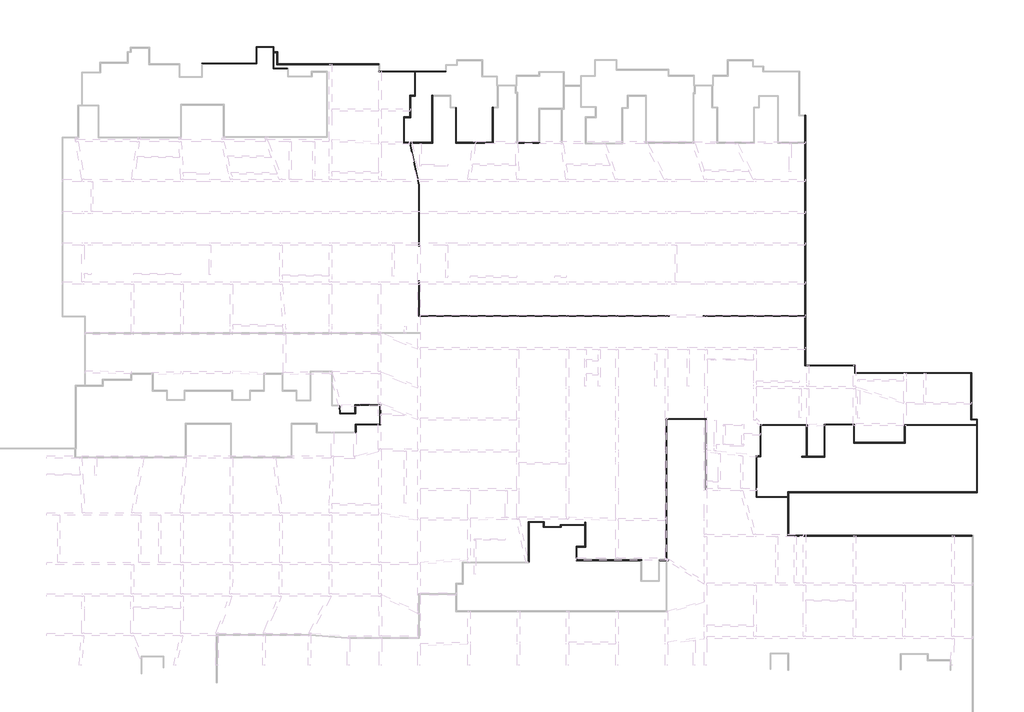
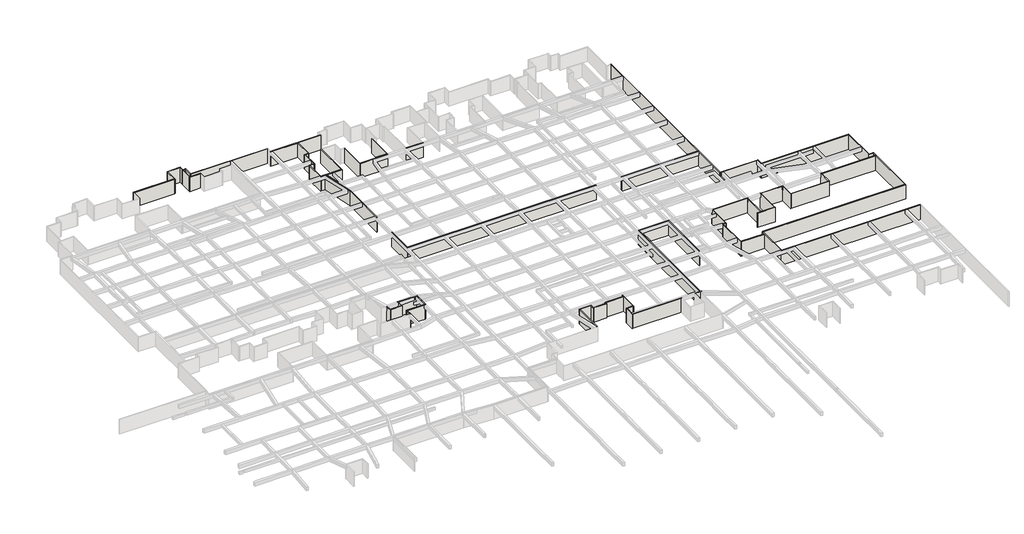
# One storey, part 4 of 16: 70 walls.
"""IFC4 building model written with IfcOpenShell, lengths in millimetres."""

from ifc_helpers import new_model, si_unit, origin, origin_with_axes, place, context, project, spatial, polyline, outline, extrude, faceted_brep, element, save

model = new_model("IFC4")

# Units and contexts
model_context = context("Model", 3, world=origin())
ifc_project = project(units=[si_unit("LENGTHUNIT", "METRE", prefix="MILLI")], contexts=[model_context])

# Site, building, storey
site = spatial("IfcSite", under=ifc_project)
building = spatial("IfcBuilding", under=site)
storey = spatial("IfcBuildingStorey", under=building, Name="户型图", Elevation=0.0)

# Walls
placement = place(None, origin())
element("IfcWall", 1, ObjectType="所有墙体", at=placement, inside=storey, context=model_context, shape_type="Brep", body=[
    faceted_brep([(231987.9308744, 132071.3072201, 0.0), (201907.9308744, 132071.3072201, 0.0), (201787.9308744, 132071.3072201, 0.0), (201787.9308744, 132071.3072201, 3300.0), (201907.9308744, 132071.3072201, 3300.0), (231987.9308744, 132071.3072201, 3300.0), (231987.9308744, 131951.3072201, 0.0), (231987.9308744, 131951.3072201, 3300.0), (201787.9308744, 131951.3072201, 3300.0), (201787.9308744, 131951.3072201, 0.0)], [[[0, 1, 2, 3, 4, 5]], [[6, 7, 8, 9]], [[2, 1, 0, 6, 9]], [[5, 4, 3, 8, 7]], [[0, 5, 7, 6]], [[3, 2, 9, 8]]]),
])
element("IfcWall", 2, ObjectType="所有墙体", at=placement, inside=storey, context=model_context, shape_type="Brep", body=[
    faceted_brep([(201907.9308744, 132071.3072201, 0.0), (201907.9308744, 139051.3072201, 0.0), (201907.9308744, 139171.3072201, 0.0), (201907.9308744, 139171.3072201, 3300.0), (201907.9308744, 139051.3072201, 3300.0), (201907.9308744, 132071.3072201, 3300.0), (201787.9308744, 132071.3072201, 0.0), (201787.9308744, 132071.3072201, 3300.0), (201787.9308744, 138272.452754, 3300.0), (201787.9308744, 138392.452754, 3300.0), (201787.9308744, 139171.3072201, 3300.0), (201787.9308744, 139171.3072201, 0.0), (201787.9308744, 138392.452754, 0.0), (201787.9308744, 138272.452754, 0.0)], [[[0, 1, 2, 3, 4, 5]], [[6, 7, 8, 9, 10, 11, 12, 13]], [[2, 1, 0, 6, 13, 12, 11]], [[5, 4, 3, 10, 9, 8, 7]], [[0, 5, 7, 6]], [[3, 2, 11, 10]]]),
])
element("IfcWall", 3, ObjectType="所有墙体", at=placement, inside=storey, context=model_context, shape_type="Brep", body=[
    faceted_brep([(201907.9308744, 139051.3072201, 0.0), (232807.9308744, 139051.3072201, 0.0), (232807.9308744, 139051.3072201, 3300.0), (201907.9308744, 139051.3072201, 3300.0), (201907.9308744, 139171.3072201, 0.0), (201907.9308744, 139171.3072201, 3300.0), (232687.9308744, 139171.3072201, 3300.0), (232807.9308744, 139171.3072201, 3300.0), (232807.9308744, 139171.3072201, 0.0), (232687.9308744, 139171.3072201, 0.0)], [[[0, 1, 2, 3]], [[4, 5, 6, 7, 8, 9]], [[1, 0, 4, 9, 8]], [[3, 2, 7, 6, 5]], [[0, 3, 5, 4]], [[2, 1, 8, 7]]]),
])
element("IfcWall", 4, ObjectType="所有墙体", at=placement, inside=storey, context=model_context, shape_type="Brep", body=[
    faceted_brep([(232807.9308744, 139171.3072201, 0.0), (232807.9308744, 151071.3072201, 0.0), (232807.9308744, 151071.3072201, 3300.0), (232807.9308744, 139171.3072201, 3300.0), (232687.9308744, 139171.3072201, 0.0), (232687.9308744, 139171.3072201, 3300.0), (232687.9308744, 150045.8384701, 3300.0), (232687.9308744, 150165.8384701, 3300.0), (232687.9308744, 150951.3072201, 3300.0), (232687.9308744, 151071.3072201, 3300.0), (232687.9308744, 151071.3072201, 0.0), (232687.9308744, 150951.3072201, 0.0), (232687.9308744, 150165.8384701, 0.0), (232687.9308744, 150045.8384701, 0.0)], [[[0, 1, 2, 3]], [[4, 5, 6, 7, 8, 9, 10, 11, 12, 13]], [[1, 0, 4, 13, 12, 11, 10]], [[3, 2, 9, 8, 7, 6, 5]], [[0, 3, 5, 4]], [[2, 1, 10, 9]]]),
])
element("IfcWall", 5, ObjectType="所有墙体", at=placement, inside=storey, context=model_context, shape_type="Brep", body=[
    faceted_brep([(232687.9308744, 151071.3072201, 0.0), (231859.0507535, 151071.3072201, 0.0), (231739.0507535, 151071.3072201, 0.0), (231739.0507535, 151071.3072201, 3300.0), (231859.0507535, 151071.3072201, 3300.0), (232687.9308744, 151071.3072201, 3300.0), (232687.9308744, 150951.3072201, 0.0), (232687.9308744, 150951.3072201, 3300.0), (231739.0507535, 150951.3072201, 3300.0), (231739.0507535, 150951.3072201, 0.0)], [[[0, 1, 2, 3, 4, 5]], [[6, 7, 8, 9]], [[2, 1, 0, 6, 9]], [[5, 4, 3, 8, 7]], [[0, 5, 7, 6]], [[3, 2, 9, 8]]]),
])
element("IfcWall", 6, ObjectType="所有墙体", at=placement, inside=storey, context=model_context, shape_type="Brep", body=[
    faceted_brep([(231859.0507535, 151071.3072201, 0.0), (231859.0507535, 158671.3072201, 0.0), (231859.0507535, 158671.3072201, 3300.0), (231859.0507535, 151071.3072201, 3300.0), (231739.0507535, 151071.3072201, 0.0), (231739.0507535, 151071.3072201, 3300.0), (231739.0507535, 158551.3072201, 3300.0), (231739.0507535, 158671.3072201, 3300.0), (231739.0507535, 158671.3072201, 0.0), (231739.0507535, 158551.3072201, 0.0)], [[[0, 1, 2, 3]], [[4, 5, 6, 7, 8, 9]], [[1, 0, 4, 9, 8]], [[3, 2, 7, 6, 5]], [[0, 3, 5, 4]], [[2, 1, 8, 7]]]),
])
element("IfcWall", 7, ObjectType="所有墙体", at=placement, inside=storey, context=model_context, shape_type="Brep", body=[
    faceted_brep([(231739.0507535, 158671.3072201, 0.0), (212859.0507535, 158671.3072201, 0.0), (212739.0507535, 158671.3072201, 0.0), (212739.0507535, 158671.3072201, 3300.0), (212859.0507535, 158671.3072201, 3300.0), (231739.0507535, 158671.3072201, 3300.0), (231739.0507535, 158551.3072201, 0.0), (231739.0507535, 158551.3072201, 3300.0), (212739.0507535, 158551.3072201, 3300.0), (212739.0507535, 158551.3072201, 0.0)], [[[0, 1, 2, 3, 4, 5]], [[6, 7, 8, 9]], [[2, 1, 0, 6, 9]], [[5, 4, 3, 8, 7]], [[0, 5, 7, 6]], [[3, 2, 9, 8]]]),
])
element("IfcWall", 8, ObjectType="所有墙体", at=placement, inside=storey, context=model_context, shape_type="Brep", body=[
    faceted_brep([(212859.0507535, 158671.3072201, 0.0), (212859.0507535, 159922.7290951, 0.0), (212859.0507535, 159922.7290951, 3300.0), (212859.0507535, 158671.3072201, 3300.0), (212739.0507535, 158671.3072201, 0.0), (212739.0507535, 158671.3072201, 3300.0), (212739.0507535, 159802.7290951, 3300.0), (212739.0507535, 159922.7290951, 3300.0), (212739.0507535, 159922.7290951, 0.0), (212739.0507535, 159802.7290951, 0.0)], [[[0, 1, 2, 3]], [[4, 5, 6, 7, 8, 9]], [[1, 0, 4, 9, 8]], [[3, 2, 7, 6, 5]], [[0, 3, 5, 4]], [[2, 1, 8, 7]]]),
])
element("IfcWall", 9, ObjectType="所有墙体", at=placement, inside=storey, context=model_context, shape_type="Brep", body=[
    faceted_brep([(212739.0507535, 159922.7290951, 0.0), (204686.5546537, 159922.7290951, 0.0), (204566.5546537, 159922.7290951, 0.0), (204566.5546537, 159922.7290951, 3300.0), (204686.5546537, 159922.7290951, 3300.0), (212739.0507535, 159922.7290951, 3300.0), (212739.0507535, 159802.7290951, 0.0), (212739.0507535, 159802.7290951, 3300.0), (204566.5546537, 159802.7290951, 3300.0), (204566.5546537, 159802.7290951, 0.0)], [[[0, 1, 2, 3, 4, 5]], [[6, 7, 8, 9]], [[2, 1, 0, 6, 9]], [[5, 4, 3, 8, 7]], [[0, 5, 7, 6]], [[3, 2, 9, 8]]]),
])
element("IfcWall", 10, ObjectType="所有墙体", at=placement, inside=storey, context=model_context, shape_type="Brep", body=[
    faceted_brep([(204686.5546537, 159922.7290951, 0.0), (204686.5546537, 200822.7290951, 0.0), (204686.5546537, 200822.7290951, 3300.0), (204686.5546537, 159922.7290951, 3300.0), (204566.5546537, 159922.7290951, 0.0), (204566.5546537, 159922.7290951, 3300.0), (204566.5546537, 167902.578939, 3300.0), (204566.5546537, 168022.578939, 3300.0), (204566.5546537, 196227.561337, 3300.0), (204566.5546537, 196347.561337, 3300.0), (204566.5546537, 200702.7290951, 3300.0), (204566.5546537, 200822.7290951, 3300.0), (204566.5546537, 200822.7290951, 0.0), (204566.5546537, 200702.7290951, 0.0), (204566.5546537, 196347.561337, 0.0), (204566.5546537, 196227.561337, 0.0), (204566.5546537, 168022.578939, 0.0), (204566.5546537, 167902.578939, 0.0)], [[[0, 1, 2, 3]], [[4, 5, 6, 7, 8, 9, 10, 11, 12, 13, 14, 15, 16, 17]], [[1, 0, 4, 17, 16, 15, 14, 13, 12]], [[3, 2, 11, 10, 9, 8, 7, 6, 5]], [[0, 3, 5, 4]], [[2, 1, 12, 11]]]),
])
element("IfcWall", 11, ObjectType="所有墙体", at=placement, inside=storey, context=model_context, shape_type="Brep", body=[
    faceted_brep([(145813.5451849, 208022.6509701, 0.0), (135026.242901, 208022.6509701, 0.0), (134906.242901, 208022.6509701, 0.0), (134906.242901, 208022.6509701, 3300.0), (135026.242901, 208022.6509701, 3300.0), (145813.5451849, 208022.6509701, 3300.0), (145813.5451849, 207902.6509701, 0.0), (145813.5451849, 207902.6509701, 3300.0), (140883.5546537, 207902.6509701, 3300.0), (140763.5546537, 207902.6509701, 3300.0), (134906.242901, 207902.6509701, 3300.0), (134906.242901, 207902.6509701, 0.0), (140763.5546537, 207902.6509701, 0.0), (140883.5546537, 207902.6509701, 0.0)], [[[0, 1, 2, 3, 4, 5]], [[6, 7, 8, 9, 10, 11, 12, 13]], [[2, 1, 0, 6, 13, 12, 11]], [[5, 4, 3, 10, 9, 8, 7]], [[0, 5, 7, 6]], [[3, 2, 11, 10]]]),
])
element("IfcWall", 12, ObjectType="所有墙体", at=placement, inside=storey, context=model_context, shape_type="Brep", body=[
    faceted_brep([(134906.242901, 209172.8384701, 0.0), (118326.242901, 209172.8384701, 0.0), (118206.242901, 209172.8384701, 0.0), (118206.242901, 209172.8384701, 3300.0), (118326.242901, 209172.8384701, 3300.0), (134906.242901, 209172.8384701, 3300.0), (134906.242901, 209052.8384701, 0.0), (134906.242901, 209052.8384701, 3300.0), (118206.242901, 209052.8384701, 3300.0), (118206.242901, 209052.8384701, 0.0)], [[[0, 1, 2, 3, 4, 5]], [[6, 7, 8, 9]], [[2, 1, 0, 6, 9]], [[5, 4, 3, 8, 7]], [[0, 5, 7, 6]], [[3, 2, 9, 8]]]),
])
element("IfcWall", 13, ObjectType="所有墙体", at=placement, inside=storey, context=model_context, shape_type="Brep", body=[
    faceted_brep([(118326.242901, 209172.8384701, 0.0), (118326.242901, 211150.6465328, 0.0), (118326.242901, 211150.6465328, 3300.0), (118326.242901, 209172.8384701, 3300.0), (118206.242901, 209172.8384701, 0.0), (118206.242901, 209172.8384701, 3300.0), (118206.242901, 211030.6465328, 3300.0), (118206.242901, 211150.6465328, 3300.0), (118206.242901, 211150.6465328, 0.0), (118206.242901, 211030.6465328, 0.0)], [[[0, 1, 2, 3]], [[4, 5, 6, 7, 8, 9]], [[1, 0, 4, 9, 8]], [[3, 2, 7, 6, 5]], [[0, 3, 5, 4]], [[2, 1, 8, 7]]]),
])
element("IfcWall", 14, ObjectType="所有墙体", at=placement, inside=storey, context=model_context, shape_type="Brep", body=[
    faceted_brep([(118206.242901, 211150.6465328, 0.0), (117726.242901, 211150.6465328, 0.0), (117606.242901, 211150.6465328, 0.0), (117606.242901, 211150.6465328, 3300.0), (117726.242901, 211150.6465328, 3300.0), (118206.242901, 211150.6465328, 3300.0), (118206.242901, 211030.6465328, 0.0), (118206.242901, 211030.6465328, 3300.0), (117723.9765287, 211030.6465328, 3300.0), (117606.242901, 211030.6465328, 3300.0), (117606.242901, 211030.6465328, 0.0), (117723.9765287, 211030.6465328, 0.0)], [[[0, 1, 2, 3, 4, 5]], [[6, 7, 8, 9, 10, 11]], [[2, 1, 0, 6, 11, 10]], [[5, 4, 3, 9, 8, 7]], [[0, 5, 7, 6]], [[3, 2, 10, 9]]]),
])
element("IfcWall", 15, ObjectType="所有墙体", at=placement, inside=storey, context=model_context, shape_type="Brep", body=[
    faceted_brep([(117726.242901, 211150.6465328, 0.0), (117726.242901, 212022.8384701, 0.0), (117726.242901, 212022.8384701, 3300.0), (117726.242901, 211150.6465328, 3300.0), (117606.242901, 211150.6465328, 0.0), (117606.242901, 211150.6465328, 3300.0), (117606.242901, 211902.8384701, 3300.0), (117606.242901, 212022.8384701, 3300.0), (117606.242901, 212022.8384701, 0.0), (117606.242901, 211902.8384701, 0.0)], [[[0, 1, 2, 3]], [[4, 5, 6, 7, 8, 9]], [[1, 0, 4, 9, 8]], [[3, 2, 7, 6, 5]], [[0, 3, 5, 4]], [[2, 1, 8, 7]]]),
])
element("IfcWall", 16, ObjectType="所有墙体", at=placement, inside=storey, context=model_context, shape_type="Brep", body=[
    faceted_brep([(117606.242901, 212022.8384701, 0.0), (114813.9765287, 212022.8384701, 0.0), (114813.9765287, 212022.8384701, 3300.0), (117606.242901, 212022.8384701, 3300.0), (117606.242901, 211902.8384701, 0.0), (117606.242901, 211902.8384701, 3300.0), (114933.9765287, 211902.8384701, 3300.0), (114813.9765287, 211902.8384701, 3300.0), (114813.9765287, 211902.8384701, 0.0), (114933.9765287, 211902.8384701, 0.0)], [[[0, 1, 2, 3]], [[4, 5, 6, 7, 8, 9]], [[1, 0, 4, 9, 8]], [[3, 2, 7, 6, 5]], [[0, 3, 5, 4]], [[2, 1, 8, 7]]]),
])
element("IfcWall", 17, ObjectType="所有墙体", at=placement, inside=storey, context=model_context, shape_type="Brep", body=[
    faceted_brep([(114813.9765287, 211902.8384701, 0.0), (114813.9765287, 209322.8384701, 0.0), (114813.9765287, 209202.8384701, 0.0), (114813.9765287, 209202.8384701, 3300.0), (114813.9765287, 209322.8384701, 3300.0), (114813.9765287, 211902.8384701, 3300.0), (114933.9765287, 211902.8384701, 0.0), (114933.9765287, 211902.8384701, 3300.0), (114933.9765287, 209202.8384701, 3300.0), (114933.9765287, 209202.8384701, 0.0)], [[[0, 1, 2, 3, 4, 5]], [[6, 7, 8, 9]], [[2, 1, 0, 6, 9]], [[5, 4, 3, 8, 7]], [[0, 5, 7, 6]], [[3, 2, 9, 8]]]),
])
element("IfcWall", 18, ObjectType="所有墙体", at=placement, inside=storey, context=model_context, shape_type="Brep", body=[
    faceted_brep([(114813.9765287, 209322.8384701, 0.0), (105913.9765287, 209322.8384701, 0.0), (105913.9765287, 209322.8384701, 3300.0), (114813.9765287, 209322.8384701, 3300.0), (114813.9765287, 209202.8384701, 0.0), (114813.9765287, 209202.8384701, 3300.0), (106033.9765287, 209202.8384701, 3300.0), (105913.9765287, 209202.8384701, 3300.0), (105913.9765287, 209202.8384701, 0.0), (106033.9765287, 209202.8384701, 0.0)], [[[0, 1, 2, 3]], [[4, 5, 6, 7, 8, 9]], [[1, 0, 4, 9, 8]], [[3, 2, 7, 6, 5]], [[0, 3, 5, 4]], [[2, 1, 8, 7]]]),
])
element("IfcWall", 19, ObjectType="所有墙体", at=placement, inside=storey, context=model_context, shape_type="Brep", body=[
    faceted_brep([(119963.9765287, 208473.0191342, 0.0), (117723.9765287, 208473.0191342, 0.0), (117603.9765287, 208473.0191342, 0.0), (117603.9765287, 208473.0191342, 3300.0), (117723.9765287, 208473.0191342, 3300.0), (119963.9765287, 208473.0191342, 3300.0), (119963.9765287, 208353.0191342, 0.0), (119963.9765287, 208353.0191342, 3300.0), (117603.9765287, 208353.0191342, 3300.0), (117603.9765287, 208353.0191342, 0.0)], [[[0, 1, 2, 3, 4, 5]], [[6, 7, 8, 9]], [[2, 1, 0, 6, 9]], [[5, 4, 3, 8, 7]], [[0, 5, 7, 6]], [[3, 2, 9, 8]]]),
])
element("IfcWall", 20, ObjectType="所有墙体", at=placement, inside=storey, context=model_context, shape_type="Brep", body=[
    faceted_brep([(117723.9765287, 208473.0191342, 0.0), (117723.9765287, 211030.6465328, 0.0), (117723.9765287, 211030.6465328, 3300.0), (117723.9765287, 208473.0191342, 3300.0), (117603.9765287, 208473.0191342, 0.0), (117603.9765287, 208473.0191342, 3300.0), (117603.9765287, 211030.6465328, 3300.0), (117603.9765287, 211030.6465328, 0.0), (117606.242901, 211030.6465328, 0.0), (117606.242901, 211030.6465328, 3300.0)], [[[0, 1, 2, 3]], [[4, 5, 6, 7]], [[1, 0, 4, 7, 8]], [[3, 2, 9, 6, 5]], [[0, 3, 5, 4]], [[2, 1, 8, 7, 6, 9]]]),
])
element("IfcWall", 21, ObjectType="所有墙体", at=placement, inside=storey, context=model_context, shape_type="Brep", body=[
    faceted_brep([(140763.5546537, 207902.6509701, 0.0), (140763.5546537, 204022.6509701, 0.0), (140763.5546537, 203902.6509701, 0.0), (140763.5546537, 203902.6509701, 3300.0), (140763.5546537, 204022.6509701, 3300.0), (140763.5546537, 207902.6509701, 3300.0), (140883.5546537, 207902.6509701, 0.0), (140883.5546537, 207902.6509701, 3300.0), (140883.5546537, 203902.6509701, 3300.0), (140883.5546537, 203902.6509701, 0.0)], [[[0, 1, 2, 3, 4, 5]], [[6, 7, 8, 9]], [[2, 1, 0, 6, 9]], [[5, 4, 3, 8, 7]], [[0, 5, 7, 6]], [[3, 2, 9, 8]]]),
])
element("IfcWall", 22, ObjectType="所有墙体", at=placement, inside=storey, context=model_context, shape_type="Brep", body=[
    faceted_brep([(140763.5546537, 204022.6509701, 0.0), (139963.5664576, 204022.6509701, 0.0), (139963.5664576, 204022.6509701, 3300.0), (140763.5546537, 204022.6509701, 3300.0), (140763.5546537, 203902.6509701, 0.0), (140763.5546537, 203902.6509701, 3300.0), (140083.5664576, 203902.6509701, 3300.0), (139963.5664576, 203902.6509701, 3300.0), (139963.5664576, 203902.6509701, 0.0), (140083.5664576, 203902.6509701, 0.0)], [[[0, 1, 2, 3]], [[4, 5, 6, 7, 8, 9]], [[1, 0, 4, 9, 8]], [[3, 2, 7, 6, 5]], [[0, 3, 5, 4]], [[2, 1, 8, 7]]]),
])
element("IfcWall", 23, ObjectType="所有墙体", at=placement, inside=storey, context=model_context, shape_type="Brep", body=[
    faceted_brep([(139963.5664576, 203902.6509701, 0.0), (139963.5664576, 200522.6509701, 0.0), (139963.5664576, 200402.6509701, 0.0), (139963.5664576, 200402.6509701, 3300.0), (139963.5664576, 200522.6509701, 3300.0), (139963.5664576, 203902.6509701, 3300.0), (140083.5664576, 203902.6509701, 0.0), (140083.5664576, 203902.6509701, 3300.0), (140083.5664576, 200402.6509701, 3300.0), (140083.5664576, 200402.6509701, 0.0)], [[[0, 1, 2, 3, 4, 5]], [[6, 7, 8, 9]], [[2, 1, 0, 6, 9]], [[5, 4, 3, 8, 7]], [[0, 5, 7, 6]], [[3, 2, 9, 8]]]),
])
element("IfcWall", 24, ObjectType="所有墙体", at=placement, inside=storey, context=model_context, shape_type="Brep", body=[
    faceted_brep([(139963.5664576, 200522.6509701, 0.0), (138963.5664576, 200522.6509701, 0.0), (138963.5664576, 200522.6509701, 3300.0), (139963.5664576, 200522.6509701, 3300.0), (139963.5664576, 200402.6509701, 0.0), (139963.5664576, 200402.6509701, 3300.0), (139083.5664576, 200402.6509701, 3300.0), (138963.5664576, 200402.6509701, 3300.0), (138963.5664576, 200402.6509701, 0.0), (139083.5664576, 200402.6509701, 0.0)], [[[0, 1, 2, 3]], [[4, 5, 6, 7, 8, 9]], [[1, 0, 4, 9, 8]], [[3, 2, 7, 6, 5]], [[0, 3, 5, 4]], [[2, 1, 8, 7]]]),
])
element("IfcWall", 25, ObjectType="所有墙体", at=placement, inside=storey, context=model_context, shape_type="Brep", body=[
    faceted_brep([(138963.5664576, 200402.6509701, 0.0), (138963.5664576, 196207.301294, 0.0), (138963.5664576, 196207.301294, 3300.0), (138963.5664576, 200402.6509701, 3300.0), (139083.5664576, 200402.6509701, 0.0), (139083.5664576, 200402.6509701, 3300.0), (139083.5664576, 196327.301294, 3300.0), (139083.5664576, 196207.301294, 3300.0), (139083.5664576, 196207.301294, 0.0), (139083.5664576, 196327.301294, 0.0)], [[[0, 1, 2, 3]], [[4, 5, 6, 7, 8, 9]], [[1, 0, 4, 9, 8]], [[3, 2, 7, 6, 5]], [[0, 3, 5, 4]], [[2, 1, 8, 7]]]),
])
element("IfcWall", 26, ObjectType="所有墙体", at=placement, inside=storey, context=model_context, shape_type="Brep", body=[
    faceted_brep([(139083.5664576, 196207.301294, 0.0), (139937.8989231, 196207.301294, 0.0), (140060.5797945, 196207.301294, 0.0), (143683.5664576, 196207.301294, 0.0), (143683.5664576, 196207.301294, 3300.0), (140060.5797945, 196207.301294, 3300.0), (139937.8989231, 196207.301294, 3300.0), (139083.5664576, 196207.301294, 3300.0), (139083.5664576, 196327.301294, 0.0), (139083.5664576, 196327.301294, 3300.0), (143563.5664576, 196327.301294, 3300.0), (143683.5664576, 196327.301294, 3300.0), (143683.5664576, 196327.301294, 0.0), (143563.5664576, 196327.301294, 0.0)], [[[0, 1, 2, 3, 4, 5, 6, 7]], [[8, 9, 10, 11, 12, 13]], [[3, 2, 1, 0, 8, 13, 12]], [[7, 6, 5, 4, 11, 10, 9]], [[0, 7, 9, 8]], [[4, 3, 12, 11]]]),
])
element("IfcWall", 27, ObjectType="所有墙体", at=placement, inside=storey, context=model_context, shape_type="Brep", body=[
    faceted_brep([(143683.5664576, 196327.301294, 0.0), (143683.5664576, 203907.301294, 0.0), (143683.5664576, 204027.301294, 0.0), (143683.5664576, 204027.301294, 3300.0), (143683.5664576, 203907.301294, 3300.0), (143683.5664576, 196327.301294, 3300.0), (143563.5664576, 196327.301294, 0.0), (143563.5664576, 196327.301294, 3300.0), (143563.5664576, 204027.301294, 3300.0), (143563.5664576, 204027.301294, 0.0)], [[[0, 1, 2, 3, 4, 5]], [[6, 7, 8, 9]], [[2, 1, 0, 6, 9]], [[5, 4, 3, 8, 7]], [[0, 5, 7, 6]], [[3, 2, 9, 8]]]),
])
element("IfcWall", 28, ObjectType="所有墙体", at=placement, inside=storey, context=model_context, shape_type="Brep", body=[
    faceted_brep([(147463.5546537, 202007.301294, 0.0), (147463.5546537, 196207.301294, 0.0), (147463.5546537, 196207.301294, 3300.0), (147463.5546537, 202007.301294, 3300.0), (147583.5546537, 202007.301294, 0.0), (147583.5546537, 202007.301294, 3300.0), (147583.5546537, 196327.301294, 3300.0), (147583.5546537, 196207.301294, 3300.0), (147583.5546537, 196207.301294, 0.0), (147583.5546537, 196327.301294, 0.0)], [[[0, 1, 2, 3]], [[4, 5, 6, 7, 8, 9]], [[1, 0, 4, 9, 8]], [[3, 2, 7, 6, 5]], [[0, 3, 5, 4]], [[2, 1, 8, 7]]]),
])
element("IfcWall", 29, ObjectType="所有墙体", at=placement, inside=storey, context=model_context, shape_type="Brep", body=[
    faceted_brep([(147583.5546537, 196207.301294, 0.0), (153583.5546537, 196207.301294, 0.0), (153583.5546537, 196207.301294, 3300.0), (147583.5546537, 196207.301294, 3300.0), (147583.5546537, 196327.301294, 0.0), (147583.5546537, 196327.301294, 3300.0), (153463.5546537, 196327.301294, 3300.0), (153583.5546537, 196327.301294, 3300.0), (153583.5546537, 196327.301294, 0.0), (153463.5546537, 196327.301294, 0.0)], [[[0, 1, 2, 3]], [[4, 5, 6, 7, 8, 9]], [[1, 0, 4, 9, 8]], [[3, 2, 7, 6, 5]], [[0, 3, 5, 4]], [[2, 1, 8, 7]]]),
])
element("IfcWall", 30, ObjectType="所有墙体", at=placement, inside=storey, context=model_context, shape_type="Brep", body=[
    faceted_brep([(153583.5546537, 196327.301294, 0.0), (153583.5546537, 202007.301294, 0.0), (153583.5546537, 202127.301294, 0.0), (153583.5546537, 202127.301294, 3300.0), (153583.5546537, 202007.301294, 3300.0), (153583.5546537, 196327.301294, 3300.0), (153463.5546537, 196327.301294, 0.0), (153463.5546537, 196327.301294, 3300.0), (153463.5546537, 202127.301294, 3300.0), (153463.5546537, 202127.301294, 0.0)], [[[0, 1, 2, 3, 4, 5]], [[6, 7, 8, 9]], [[2, 1, 0, 6, 9]], [[5, 4, 3, 8, 7]], [[0, 5, 7, 6]], [[3, 2, 9, 8]]]),
])
element("IfcWall", 31, ObjectType="所有墙体", at=placement, inside=storey, context=model_context, shape_type="Brep", body=[
    faceted_brep([(157583.5564847, 196202.6509701, 0.0), (161183.5564847, 196202.6509701, 0.0), (161183.5564847, 196202.6509701, 3300.0), (157583.5564847, 196202.6509701, 3300.0), (157583.5564847, 196322.6509701, 0.0), (157583.5564847, 196322.6509701, 3300.0), (161063.5564847, 196322.6509701, 3300.0), (161183.5564847, 196322.6509701, 3300.0), (161183.5564847, 196322.6509701, 0.0), (161063.5564847, 196322.6509701, 0.0)], [[[0, 1, 2, 3]], [[4, 5, 6, 7, 8, 9]], [[1, 0, 4, 9, 8]], [[3, 2, 7, 6, 5]], [[0, 3, 5, 4]], [[2, 1, 8, 7]]]),
])
element("IfcWall", 32, ObjectType="所有墙体", at=placement, inside=storey, context=model_context, shape_type="SweptSolid", body=[
    extrude(outline(polyline([(141400.1899051, 189327.7631113), (139937.8989231, 196207.301294), (140060.5797945, 196207.301294), (141520.1899051, 189340.3756196), (141400.1899051, 189327.7631113)])), origin_with_axes(), (0.0, 0.0, 1.0), 3300.0),
])
element("IfcWall", 33, ObjectType="所有墙体", at=placement, inside=storey, context=model_context, shape_type="SweptSolid", body=[
    extrude(outline(polyline([(141400.1899051, 179334.0693654), (141400.1899051, 189327.7631113), (141520.1899051, 189340.3756196), (141520.1899051, 179334.0693654), (141400.1899051, 179334.0693654)])), origin_with_axes(), (0.0, 0.0, 1.0), 3300.0),
])
element("IfcWall", 34, ObjectType="所有墙体", at=placement, inside=storey, context=model_context, shape_type="Brep", body=[
    faceted_brep([(141406.2091209, 173712.5789366, 0.0), (141406.2091209, 167902.578939, 0.0), (141406.2091209, 167902.578939, 3300.0), (141406.2091209, 173712.5789366, 3300.0), (141526.2091209, 173712.5789366, 0.0), (141526.2091209, 173712.5789366, 3300.0), (141526.2091209, 168022.578939, 3300.0), (141526.2091209, 167902.578939, 3300.0), (141526.2091209, 167902.578939, 0.0), (141526.2091209, 168022.578939, 0.0)], [[[0, 1, 2, 3]], [[4, 5, 6, 7, 8, 9]], [[1, 0, 4, 9, 8]], [[3, 2, 7, 6, 5]], [[0, 3, 5, 4]], [[2, 1, 8, 7]]]),
])
element("IfcWall", 35, ObjectType="所有墙体", at=placement, inside=storey, context=model_context, shape_type="SweptSolid", body=[
    extrude(outline(polyline([(182416.2091202, 167902.578939), (141526.2091209, 167902.578939), (141526.2091209, 168022.578939), (182416.2091202, 168022.578939), (182416.2091202, 167902.578939)])), origin_with_axes(), (0.0, 0.0, 1.0), 3300.0),
])
element("IfcWall", 36, ObjectType="所有墙体", at=placement, inside=storey, context=model_context, shape_type="SweptSolid", body=[
    extrude(outline(polyline([(204566.5546537, 167902.578939), (187916.2091202, 167902.578939), (187916.2091202, 168022.578939), (204566.5546537, 168022.578939), (204566.5546537, 167902.578939)])), origin_with_axes(), (0.0, 0.0, 1.0), 3300.0),
])
element("IfcWall", 37, ObjectType="所有墙体", at=placement, inside=storey, context=model_context, shape_type="Brep", body=[
    faceted_brep([(128415.7648004, 153225.3546981, 0.0), (128489.0373514, 151924.651075, 0.0), (128489.0373514, 151924.651075, 3300.0), (128415.7648004, 153225.3546981, 3300.0), (128535.9550541, 153225.3546981, 0.0), (128535.9550541, 153225.3546981, 3300.0), (128602.4676438, 152044.651075, 3300.0), (128609.2276051, 151924.651075, 3300.0), (128609.2276051, 151924.651075, 0.0), (128602.4676438, 152044.651075, 0.0)], [[[0, 1, 2, 3]], [[4, 5, 6, 7, 8, 9]], [[1, 0, 4, 9, 8]], [[3, 2, 7, 6, 5]], [[0, 3, 5, 4]], [[2, 1, 8, 7]]]),
])
element("IfcWall", 38, ObjectType="所有墙体", at=placement, inside=storey, context=model_context, shape_type="Brep", body=[
    faceted_brep([(128609.2276051, 151924.651075, 0.0), (131082.4811371, 151924.651075, 0.0), (131082.4811371, 151924.651075, 3300.0), (128609.2276051, 151924.651075, 3300.0), (128602.4676438, 152044.651075, 0.0), (128602.4676438, 152044.651075, 3300.0), (130962.4811371, 152044.651075, 3300.0), (131082.4811371, 152044.651075, 3300.0), (131082.4811371, 152044.651075, 0.0), (130962.4811371, 152044.651075, 0.0)], [[[0, 1, 2, 3]], [[4, 5, 6, 7, 8, 9]], [[1, 0, 4, 9, 8]], [[3, 2, 7, 6, 5]], [[0, 3, 5, 4]], [[2, 1, 8, 7]]]),
])
element("IfcWall", 39, ObjectType="所有墙体", at=placement, inside=storey, context=model_context, shape_type="Brep", body=[
    faceted_brep([(131082.4811371, 152044.651075, 0.0), (131082.4811371, 153349.6509701, 0.0), (131082.4811371, 153469.6509701, 0.0), (131082.4811371, 153469.6509701, 3300.0), (131082.4811371, 153349.6509701, 3300.0), (131082.4811371, 152044.651075, 3300.0), (130962.4811371, 152044.651075, 0.0), (130962.4811371, 152044.651075, 3300.0), (130962.4811371, 153469.6509701, 3300.0), (130962.4811371, 153469.6509701, 0.0)], [[[0, 1, 2, 3, 4, 5]], [[6, 7, 8, 9]], [[2, 1, 0, 6, 9]], [[5, 4, 3, 8, 7]], [[0, 5, 7, 6]], [[3, 2, 9, 8]]]),
])
element("IfcWall", 40, ObjectType="所有墙体", at=placement, inside=storey, context=model_context, shape_type="Brep", body=[
    faceted_brep([(131082.4811371, 153349.6509701, 0.0), (135042.4811371, 153349.6509701, 0.0), (135162.4811371, 153349.6509701, 0.0), (135162.4811371, 153349.6509701, 3300.0), (135042.4811371, 153349.6509701, 3300.0), (131082.4811371, 153349.6509701, 3300.0), (131082.4811371, 153469.6509701, 0.0), (131082.4811371, 153469.6509701, 3300.0), (135162.4811371, 153469.6509701, 3300.0), (135162.4811371, 153469.6509701, 0.0)], [[[0, 1, 2, 3, 4, 5]], [[6, 7, 8, 9]], [[2, 1, 0, 6, 9]], [[5, 4, 3, 8, 7]], [[0, 5, 7, 6]], [[3, 2, 9, 8]]]),
])
element("IfcWall", 41, ObjectType="所有墙体", at=placement, inside=storey, context=model_context, shape_type="Brep", body=[
    faceted_brep([(135042.4811371, 153349.6509701, 0.0), (135042.4811371, 150244.6509701, 0.0), (135042.4811371, 150124.6509701, 0.0), (135042.4811371, 150124.6509701, 3300.0), (135042.4811371, 150244.6509701, 3300.0), (135042.4811371, 153349.6509701, 3300.0), (135162.4811371, 153349.6509701, 0.0), (135162.4811371, 153349.6509701, 3300.0), (135162.4811371, 150124.6509701, 3300.0), (135162.4811371, 150124.6509701, 0.0)], [[[0, 1, 2, 3, 4, 5]], [[6, 7, 8, 9]], [[2, 1, 0, 6, 9]], [[5, 4, 3, 8, 7]], [[0, 5, 7, 6]], [[3, 2, 9, 8]]]),
])
element("IfcWall", 42, ObjectType="所有墙体", at=placement, inside=storey, context=model_context, shape_type="Brep", body=[
    faceted_brep([(135042.4811371, 150244.6509701, 0.0), (131062.4799466, 150244.6509701, 0.0), (131062.4799466, 150244.6509701, 3300.0), (135042.4811371, 150244.6509701, 3300.0), (135042.4811371, 150124.6509701, 0.0), (135042.4811371, 150124.6509701, 3300.0), (131182.4799466, 150124.6509701, 3300.0), (131062.4799466, 150124.6509701, 3300.0), (131062.4799466, 150124.6509701, 0.0), (131182.4799466, 150124.6509701, 0.0)], [[[0, 1, 2, 3]], [[4, 5, 6, 7, 8, 9]], [[1, 0, 4, 9, 8]], [[3, 2, 7, 6, 5]], [[0, 3, 5, 4]], [[2, 1, 8, 7]]]),
])
element("IfcWall", 43, ObjectType="所有墙体", at=placement, inside=storey, context=model_context, shape_type="Brep", body=[
    faceted_brep([(131062.4799466, 150124.6509701, 0.0), (131062.4799466, 148944.6509701, 0.0), (131062.4799466, 148824.6509701, 0.0), (131062.4799466, 148824.6509701, 3300.0), (131062.4799466, 148944.6509701, 3300.0), (131062.4799466, 150124.6509701, 3300.0), (131182.4799466, 150124.6509701, 0.0), (131182.4799466, 150124.6509701, 3300.0), (131182.4799466, 148824.6509701, 3300.0), (131182.4799466, 148824.6509701, 0.0)], [[[0, 1, 2, 3, 4, 5]], [[6, 7, 8, 9]], [[2, 1, 0, 6, 9]], [[5, 4, 3, 8, 7]], [[0, 5, 7, 6]], [[3, 2, 9, 8]]]),
])
element("IfcWall", 44, ObjectType="所有墙体", at=placement, inside=storey, context=model_context, shape_type="Brep", body=[
    faceted_brep([(159343.2890287, 134178.5789365, 0.0), (159463.2890287, 134178.5789365, 0.0), (161793.3937956, 134178.5789365, 0.0), (161913.3937956, 134178.5789365, 0.0), (161913.3937956, 134178.5789365, 3300.0), (161793.3937956, 134178.5789365, 3300.0), (159463.2890287, 134178.5789365, 3300.0), (159343.2890287, 134178.5789365, 3300.0), (159343.2890287, 134298.5789365, 0.0), (159343.2890287, 134298.5789365, 3300.0), (161913.3937956, 134298.5789365, 3300.0), (161913.3937956, 134298.5789365, 0.0)], [[[0, 1, 2, 3, 4, 5, 6, 7]], [[8, 9, 10, 11]], [[3, 2, 1, 0, 8, 11]], [[7, 6, 5, 4, 10, 9]], [[4, 3, 11, 10]], [[0, 7, 9, 8]]]),
])
element("IfcWall", 45, ObjectType="所有墙体", at=placement, inside=storey, context=model_context, shape_type="Brep", body=[
    faceted_brep([(161793.3937956, 134178.5789365, 0.0), (161793.3937956, 133378.1355885, 0.0), (161793.3937956, 133378.1355885, 3300.0), (161793.3937956, 134178.5789365, 3300.0), (161913.3937956, 134178.5789365, 0.0), (161913.3937956, 134178.5789365, 3300.0), (161913.3937956, 133498.1355885, 3300.0), (161913.3937956, 133378.1355885, 3300.0), (161913.3937956, 133378.1355885, 0.0), (161913.3937956, 133498.1355885, 0.0)], [[[0, 1, 2, 3]], [[4, 5, 6, 7, 8, 9]], [[1, 0, 4, 9, 8]], [[3, 2, 7, 6, 5]], [[0, 3, 5, 4]], [[2, 1, 8, 7]]]),
])
element("IfcWall", 46, ObjectType="所有墙体", at=placement, inside=storey, context=model_context, shape_type="Brep", body=[
    faceted_brep([(161913.3937956, 133378.1355885, 0.0), (164713.3699471, 133378.1355885, 0.0), (164713.3699471, 133378.1355885, 3300.0), (161913.3937956, 133378.1355885, 3300.0), (161913.3937956, 133498.1355885, 0.0), (161913.3937956, 133498.1355885, 3300.0), (164593.3699471, 133498.1355885, 3300.0), (164713.3699471, 133498.1355885, 3300.0), (164713.3699471, 133498.1355885, 0.0), (164593.3699471, 133498.1355885, 0.0)], [[[0, 1, 2, 3]], [[4, 5, 6, 7, 8, 9]], [[1, 0, 4, 9, 8]], [[3, 2, 7, 6, 5]], [[0, 3, 5, 4]], [[2, 1, 8, 7]]]),
])
element("IfcWall", 47, ObjectType="所有墙体", at=placement, inside=storey, context=model_context, shape_type="Brep", body=[
    faceted_brep([(164713.3699471, 133498.1355885, 0.0), (164713.3699471, 133702.5789365, 0.0), (164713.3699471, 133822.5789365, 0.0), (164713.3699471, 133822.5789365, 3300.0), (164713.3699471, 133702.5789365, 3300.0), (164713.3699471, 133498.1355885, 3300.0), (164593.3699471, 133498.1355885, 0.0), (164593.3699471, 133498.1355885, 3300.0), (164593.3699471, 133822.5789365, 3300.0), (164593.3699471, 133822.5789365, 0.0)], [[[0, 1, 2, 3, 4, 5]], [[6, 7, 8, 9]], [[2, 1, 0, 6, 9]], [[5, 4, 3, 8, 7]], [[0, 5, 7, 6]], [[3, 2, 9, 8]]]),
])
element("IfcWall", 48, ObjectType="所有墙体", at=placement, inside=storey, context=model_context, shape_type="SweptSolid", body=[
    extrude(outline(polyline([(168593.4462779, 133702.5789365), (164713.3699471, 133702.5789365), (164713.3699471, 133822.5789365), (168593.4462779, 133822.5789365), (168593.4462779, 133702.5789365)])), origin_with_axes(), (0.0, 0.0, 1.0), 3300.0),
])
element("IfcWall", 49, ObjectType="所有墙体", at=placement, inside=storey, context=model_context, shape_type="Brep", body=[
    faceted_brep([(168713.4462779, 130128.0259701, 0.0), (168713.4462779, 134238.5789365, 0.0), (168713.4462779, 134238.5789365, 3300.0), (168713.4462779, 130128.0259701, 3300.0), (168593.4462779, 130128.0259701, 0.0), (168593.4462779, 130128.0259701, 3300.0), (168593.4462779, 130248.0259701, 3300.0), (168593.4462779, 133702.5789365, 3300.0), (168593.4462779, 133822.5789365, 3300.0), (168593.4462779, 134238.5789365, 3300.0), (168593.4462779, 134238.5789365, 0.0), (168593.4462779, 133822.5789365, 0.0), (168593.4462779, 133702.5789365, 0.0), (168593.4462779, 130248.0259701, 0.0)], [[[0, 1, 2, 3]], [[4, 5, 6, 7, 8, 9, 10, 11, 12, 13]], [[1, 0, 4, 13, 12, 11, 10]], [[2, 1, 10, 9]], [[3, 2, 9, 8, 7, 6, 5]], [[0, 3, 5, 4]]]),
])
element("IfcWall", 50, ObjectType="所有墙体", at=placement, inside=storey, context=model_context, shape_type="Brep", body=[
    faceted_brep([(168593.4462779, 130248.0259701, 0.0), (167143.2890287, 130248.0259701, 0.0), (167143.2890287, 130248.0259701, 3300.0), (168593.4462779, 130248.0259701, 3300.0), (168593.4462779, 130128.0259701, 0.0), (168593.4462779, 130128.0259701, 3300.0), (167263.2890287, 130128.0259701, 3300.0), (167143.2890287, 130128.0259701, 3300.0), (167143.2890287, 130128.0259701, 0.0), (167263.2890287, 130128.0259701, 0.0)], [[[0, 1, 2, 3]], [[4, 5, 6, 7, 8, 9]], [[1, 0, 4, 9, 8]], [[3, 2, 7, 6, 5]], [[0, 3, 5, 4]], [[2, 1, 8, 7]]]),
])
element("IfcWall", 51, ObjectType="所有墙体", at=placement, inside=storey, context=model_context, shape_type="Brep", body=[
    faceted_brep([(167143.2890287, 130128.0259701, 0.0), (167143.2890287, 127952.5884701, 0.0), (167143.2890287, 127952.5884701, 3300.0), (167143.2890287, 130128.0259701, 3300.0), (167263.2890287, 130128.0259701, 0.0), (167263.2890287, 130128.0259701, 3300.0), (167263.2890287, 128072.5884701, 3300.0), (167263.2890287, 127952.5884701, 3300.0), (167263.2890287, 127952.5884701, 0.0), (167263.2890287, 128072.5884701, 0.0)], [[[0, 1, 2, 3]], [[4, 5, 6, 7, 8, 9]], [[1, 0, 4, 9, 8]], [[3, 2, 7, 6, 5]], [[0, 3, 5, 4]], [[2, 1, 8, 7]]]),
])
element("IfcWall", 52, ObjectType="所有墙体", at=placement, inside=storey, context=model_context, shape_type="Brep", body=[
    faceted_brep([(167263.2890287, 127952.5884701, 0.0), (177743.2890287, 127952.5884701, 0.0), (177863.2890287, 127952.5884701, 0.0), (177863.2890287, 127952.5884701, 3300.0), (177743.2890287, 127952.5884701, 3300.0), (167263.2890287, 127952.5884701, 3300.0), (167263.2890287, 128072.5884701, 0.0), (167263.2890287, 128072.5884701, 3300.0), (177863.2890287, 128072.5884701, 3300.0), (177863.2890287, 128072.5884701, 0.0)], [[[0, 1, 2, 3, 4, 5]], [[6, 7, 8, 9]], [[2, 1, 0, 6, 9]], [[5, 4, 3, 8, 7]], [[0, 5, 7, 6]], [[3, 2, 9, 8]]]),
])
element("IfcWall", 53, ObjectType="所有墙体", at=placement, inside=storey, context=model_context, shape_type="Brep", body=[
    faceted_brep([(180763.3460986, 127952.5884701, 0.0), (181897.7367524, 127952.5884701, 0.0), (182017.7367524, 127952.5884701, 0.0), (182216.2109037, 127952.5884701, 0.0), (182216.2109037, 127952.5884701, 3300.0), (182017.7367524, 127952.5884701, 3300.0), (181897.7367524, 127952.5884701, 3300.0), (180763.3460986, 127952.5884701, 3300.0), (180763.3460986, 128072.5884701, 0.0), (180763.3460986, 128072.5884701, 3300.0), (182216.2109037, 128072.5884701, 3300.0), (182216.2109037, 128072.5884701, 0.0)], [[[0, 1, 2, 3, 4, 5, 6, 7]], [[8, 9, 10, 11]], [[3, 2, 1, 0, 8, 11]], [[4, 3, 11, 10]], [[7, 6, 5, 4, 10, 9]], [[0, 7, 9, 8]]]),
])
element("IfcWall", 54, ObjectType="所有墙体", at=placement, inside=storey, context=model_context, shape_type="SweptSolid", body=[
    extrude(outline(polyline([(159463.2890287, 134178.5789365), (159463.2890287, 127698.0259701), (159343.2890287, 127698.0259701), (159343.2890287, 134178.5789365), (159463.2890287, 134178.5789365)])), origin_with_axes(), (0.0, 0.0, 1.0), 3300.0),
])
element("IfcWall", 55, ObjectType="所有墙体", at=placement, inside=storey, context=model_context, shape_type="Brep", body=[
    faceted_brep([(204959.2888734, 150165.8384701, 0.0), (197239.2888734, 150165.8384701, 0.0), (197239.2888734, 150165.8384701, 3300.0), (204959.2888734, 150165.8384701, 3300.0), (204959.2888734, 150045.8384701, 0.0), (204959.2888734, 150045.8384701, 3300.0), (204839.2888734, 150045.8384701, 3300.0), (197359.2888734, 150045.8384701, 3300.0), (197239.2888734, 150045.8384701, 3300.0), (197239.2888734, 150045.8384701, 0.0), (197359.2888734, 150045.8384701, 0.0), (204839.2888734, 150045.8384701, 0.0)], [[[0, 1, 2, 3]], [[4, 5, 6, 7, 8, 9, 10, 11]], [[1, 0, 4, 11, 10, 9]], [[3, 2, 8, 7, 6, 5]], [[2, 1, 9, 8]], [[0, 3, 5, 4]]]),
])
element("IfcWall", 56, ObjectType="所有墙体", at=placement, inside=storey, context=model_context, shape_type="Brep", body=[
    faceted_brep([(197239.2888734, 150045.8384701, 0.0), (197239.2888734, 145065.8384701, 0.0), (197239.2888734, 144945.8384701, 0.0), (197239.2888734, 144945.8384701, 3300.0), (197239.2888734, 145065.8384701, 3300.0), (197239.2888734, 150045.8384701, 3300.0), (197359.2888734, 150045.8384701, 0.0), (197359.2888734, 150045.8384701, 3300.0), (197359.2888734, 144945.8384701, 3300.0), (197359.2888734, 144945.8384701, 0.0)], [[[0, 1, 2, 3, 4, 5]], [[6, 7, 8, 9]], [[2, 1, 0, 6, 9]], [[5, 4, 3, 8, 7]], [[0, 5, 7, 6]], [[3, 2, 9, 8]]]),
])
element("IfcWall", 57, ObjectType="所有墙体", at=placement, inside=storey, context=model_context, shape_type="Brep", body=[
    faceted_brep([(197239.2888734, 145065.8384701, 0.0), (196606.2109037, 145065.8384701, 0.0), (196606.2109037, 145065.8384701, 3300.0), (197239.2888734, 145065.8384701, 3300.0), (197239.2888734, 144945.8384701, 0.0), (197239.2888734, 144945.8384701, 3300.0), (196726.2109037, 144945.8384701, 3300.0), (196606.2109037, 144945.8384701, 3300.0), (196606.2109037, 144945.8384701, 0.0), (196726.2109037, 144945.8384701, 0.0)], [[[0, 1, 2, 3]], [[4, 5, 6, 7, 8, 9]], [[1, 0, 4, 9, 8]], [[3, 2, 7, 6, 5]], [[0, 3, 5, 4]], [[2, 1, 8, 7]]]),
])
element("IfcWall", 58, ObjectType="所有墙体", at=placement, inside=storey, context=model_context, shape_type="Brep", body=[
    faceted_brep([(196606.2109037, 144945.8384701, 0.0), (196606.2109037, 138272.452754, 0.0), (196606.2109037, 138272.452754, 3300.0), (196606.2109037, 144945.8384701, 3300.0), (196726.2109037, 144945.8384701, 0.0), (196726.2109037, 144945.8384701, 3300.0), (196726.2109037, 138392.452754, 3300.0), (196726.2109037, 138272.452754, 3300.0), (196726.2109037, 138272.452754, 0.0), (196726.2109037, 138392.452754, 0.0)], [[[0, 1, 2, 3]], [[4, 5, 6, 7, 8, 9]], [[1, 0, 4, 9, 8]], [[3, 2, 7, 6, 5]], [[0, 3, 5, 4]], [[2, 1, 8, 7]]]),
])
element("IfcWall", 59, ObjectType="所有墙体", at=placement, inside=storey, context=model_context, shape_type="SweptSolid", body=[
    extrude(outline(polyline([(201787.9308744, 138272.452754), (196726.2109037, 138272.452754), (196726.2109037, 138392.452754), (201787.9308744, 138392.452754), (201787.9308744, 138272.452754)])), origin_with_axes(), (0.0, 0.0, 1.0), 3300.0),
])
element("IfcWall", 60, ObjectType="所有墙体", at=placement, inside=storey, context=model_context, shape_type="SweptSolid", body=[
    extrude(outline(polyline([(204839.2888734, 144965.8384701), (204839.2888734, 150045.8384701), (204959.2888734, 150045.8384701), (204959.2888734, 144965.8384701), (204839.2888734, 144965.8384701)])), origin_with_axes(), (0.0, 0.0, 1.0), 3300.0),
])
element("IfcWall", 61, ObjectType="所有墙体", at=placement, inside=storey, context=model_context, shape_type="Brep", body=[
    faceted_brep([(207859.2888734, 144965.8384701, 0.0), (207739.2888734, 144965.8384701, 0.0), (204959.2888734, 144965.8384701, 0.0), (204839.2888734, 144965.8384701, 0.0), (204099.2888734, 144965.8384701, 0.0), (204099.2888734, 144965.8384701, 3300.0), (204839.2888734, 144965.8384701, 3300.0), (204959.2888734, 144965.8384701, 3300.0), (207739.2888734, 144965.8384701, 3300.0), (207859.2888734, 144965.8384701, 3300.0), (207859.2888734, 144845.8384701, 0.0), (207859.2888734, 144845.8384701, 3300.0), (204099.2888734, 144845.8384701, 3300.0), (204099.2888734, 144845.8384701, 0.0)], [[[0, 1, 2, 3, 4, 5, 6, 7, 8, 9]], [[10, 11, 12, 13]], [[4, 3, 2, 1, 0, 10, 13]], [[5, 4, 13, 12]], [[9, 8, 7, 6, 5, 12, 11]], [[0, 9, 11, 10]]]),
])
element("IfcWall", 62, ObjectType="所有墙体", at=placement, inside=storey, context=model_context, shape_type="Brep", body=[
    faceted_brep([(207859.2888734, 144965.8384701, 0.0), (207859.2888734, 150145.8384701, 0.0), (207859.2888734, 150265.8384701, 0.0), (207859.2888734, 150265.8384701, 3300.0), (207859.2888734, 150145.8384701, 3300.0), (207859.2888734, 144965.8384701, 3300.0), (207739.2888734, 144965.8384701, 0.0), (207739.2888734, 144965.8384701, 3300.0), (207739.2888734, 150265.8384701, 3300.0), (207739.2888734, 150265.8384701, 0.0)], [[[0, 1, 2, 3, 4, 5]], [[6, 7, 8, 9]], [[2, 1, 0, 6, 9]], [[5, 4, 3, 8, 7]], [[0, 5, 7, 6]], [[3, 2, 9, 8]]]),
])
element("IfcWall", 63, ObjectType="所有墙体", at=placement, inside=storey, context=model_context, shape_type="Brep", body=[
    faceted_brep([(207859.2888734, 150145.8384701, 0.0), (212539.2888734, 150145.8384701, 0.0), (212659.2888734, 150145.8384701, 0.0), (212659.2888734, 150145.8384701, 3300.0), (212539.2888734, 150145.8384701, 3300.0), (207859.2888734, 150145.8384701, 3300.0), (207859.2888734, 150265.8384701, 0.0), (207859.2888734, 150265.8384701, 3300.0), (212659.2888734, 150265.8384701, 3300.0), (212659.2888734, 150265.8384701, 0.0)], [[[0, 1, 2, 3, 4, 5]], [[6, 7, 8, 9]], [[2, 1, 0, 6, 9]], [[5, 4, 3, 8, 7]], [[0, 5, 7, 6]], [[3, 2, 9, 8]]]),
])
element("IfcWall", 64, ObjectType="所有墙体", at=placement, inside=storey, context=model_context, shape_type="Brep", body=[
    faceted_brep([(212539.2888734, 150145.8384701, 0.0), (212539.2888734, 147145.8384701, 0.0), (212539.2888734, 147145.8384701, 3300.0), (212539.2888734, 150145.8384701, 3300.0), (212659.2888734, 150145.8384701, 0.0), (212659.2888734, 150145.8384701, 3300.0), (212659.2888734, 147265.8384701, 3300.0), (212659.2888734, 147145.8384701, 3300.0), (212659.2888734, 147145.8384701, 0.0), (212659.2888734, 147265.8384701, 0.0)], [[[0, 1, 2, 3]], [[4, 5, 6, 7, 8, 9]], [[1, 0, 4, 9, 8]], [[3, 2, 7, 6, 5]], [[0, 3, 5, 4]], [[2, 1, 8, 7]]]),
])
element("IfcWall", 65, ObjectType="所有墙体", at=placement, inside=storey, context=model_context, shape_type="Brep", body=[
    faceted_brep([(212659.2888734, 147145.8384701, 0.0), (220959.2888734, 147145.8384701, 0.0), (220959.2888734, 147145.8384701, 3300.0), (212659.2888734, 147145.8384701, 3300.0), (212659.2888734, 147265.8384701, 0.0), (212659.2888734, 147265.8384701, 3300.0), (220839.2888734, 147265.8384701, 3300.0), (220959.2888734, 147265.8384701, 3300.0), (220959.2888734, 147265.8384701, 0.0), (220839.2888734, 147265.8384701, 0.0)], [[[0, 1, 2, 3]], [[4, 5, 6, 7, 8, 9]], [[1, 0, 4, 9, 8]], [[3, 2, 7, 6, 5]], [[0, 3, 5, 4]], [[2, 1, 8, 7]]]),
])
element("IfcWall", 66, ObjectType="所有墙体", at=placement, inside=storey, context=model_context, shape_type="Brep", body=[
    faceted_brep([(220959.2888734, 147265.8384701, 0.0), (220959.2888734, 150045.8384701, 0.0), (220959.2888734, 150165.8384701, 0.0), (220959.2888734, 150165.8384701, 3300.0), (220959.2888734, 150045.8384701, 3300.0), (220959.2888734, 147265.8384701, 3300.0), (220839.2888734, 147265.8384701, 0.0), (220839.2888734, 147265.8384701, 3300.0), (220839.2888734, 150165.8384701, 3300.0), (220839.2888734, 150165.8384701, 0.0)], [[[0, 1, 2, 3, 4, 5]], [[6, 7, 8, 9]], [[2, 1, 0, 6, 9]], [[5, 4, 3, 8, 7]], [[0, 5, 7, 6]], [[3, 2, 9, 8]]]),
])
element("IfcWall", 67, ObjectType="所有墙体", at=placement, inside=storey, context=model_context, shape_type="SweptSolid", body=[
    extrude(outline(polyline([(232687.9308744, 150045.8384701), (220959.2888734, 150045.8384701), (220959.2888734, 150165.8384701), (232687.9308744, 150165.8384701), (232687.9308744, 150045.8384701)])), origin_with_axes(), (0.0, 0.0, 1.0), 3300.0),
])
element("IfcWall", 68, ObjectType="所有墙体", at=placement, inside=storey, context=model_context, shape_type="Brep", body=[
    faceted_brep([(182017.7367524, 128072.5884701, 0.0), (182017.7367524, 151052.5884701, 0.0), (182017.7367524, 151172.5884701, 0.0), (182017.7367524, 151172.5884701, 3300.0), (182017.7367524, 151052.5884701, 3300.0), (182017.7367524, 128212.6640931, 3300.0), (182017.7367524, 128072.5884701, 3300.0), (182017.7367524, 128072.5884701, 2500.0), (181897.7367524, 128072.5884701, 0.0), (181897.7367524, 128072.5884701, 2500.0), (181897.7367524, 128072.5884701, 3300.0), (181897.7367524, 128212.6640931, 3300.0), (181897.7367524, 151172.5884701, 3300.0), (181897.7367524, 151172.5884701, 2500.0), (181897.7367524, 151172.5884701, 0.0)], [[[0, 1, 2, 3, 4, 5, 6, 7]], [[8, 9, 10, 11, 12, 13, 14]], [[2, 1, 0, 8, 14]], [[6, 5, 4, 3, 12, 11, 10]], [[0, 7, 6, 10, 9, 8]], [[3, 2, 14, 13, 12]]]),
])
element("IfcWall", 69, ObjectType="所有墙体", at=placement, inside=storey, context=model_context, shape_type="Brep", body=[
    faceted_brep([(182017.7367524, 151052.5884701, 0.0), (188356.2109037, 151052.5884701, 0.0), (188356.2109037, 151052.5884701, 2500.0), (188356.2109037, 151052.5884701, 3300.0), (182116.2109037, 151052.5884701, 3300.0), (182017.7367524, 151052.5884701, 3300.0), (182017.7367524, 151052.5884701, 2500.0), (182017.7367524, 151172.5884701, 0.0), (182017.7367524, 151172.5884701, 3300.0), (182116.2109037, 151172.5884701, 3300.0), (188356.2109037, 151172.5884701, 3300.0), (188356.2109037, 151172.5884701, 0.0)], [[[0, 1, 2, 3, 4, 5, 6]], [[7, 8, 9, 10, 11]], [[1, 0, 7, 11]], [[5, 4, 3, 10, 9, 8]], [[0, 6, 5, 8, 7]], [[3, 2, 1, 11, 10]]]),
])
element("IfcWall", 70, ObjectType="所有墙体", at=placement, inside=storey, context=model_context, shape_type="Brep", body=[
    faceted_brep([(188356.2109037, 151172.5884701, 0.0), (188356.2109037, 151052.5884701, 0.0), (188356.2109037, 139562.5884701, 0.0), (188356.2109037, 139562.5884701, 2500.0), (188356.2109037, 139562.5884701, 3300.0), (188356.2109037, 150902.424794, 3300.0), (188356.2109037, 151052.5884701, 3300.0), (188356.2109037, 151172.5884701, 3300.0), (188476.2109037, 151172.5884701, 0.0), (188476.2109037, 151172.5884701, 2500.0), (188476.2109037, 151172.5884701, 3300.0), (188476.2109037, 150902.424794, 3300.0), (188476.2109037, 139562.5884701, 3300.0), (188476.2109037, 139562.5884701, 2500.0), (188476.2109037, 139562.5884701, 0.0)], [[[0, 1, 2, 3, 4, 5, 6, 7]], [[8, 9, 10, 11, 12, 13, 14]], [[2, 1, 0, 8, 14]], [[4, 3, 2, 14, 13, 12]], [[7, 6, 5, 4, 12, 11, 10]], [[0, 7, 10, 9, 8]]]),
])

save(model, "model.ifc")

# Revit data of these elements
# Type "所有墙体"
#   Layers, outside or top first: 120 mm "默认" (function 1)
# Elements 1, 2, 3, 4, 5, 6, 7, 8, 9, 10, 11, 12, 13, 14, 15, 16, 17, 18, 19, 20, 21, 22, 23, 24, 25, 26, 27, 28, 29, 30, 31, 32, 33, 34, 35, 36, 37, 38, 39, 40, 41, 42, 43, 44, 45, 46, 47, 48, 49, 50, 51, 52, 53, 54, 55, 56, 57, 58, 59, 60, 61, 62, 63, 64, 65, 66, 67 (IfcWall, "所有墙体")
#   Top Offset = 0 mm
#   Base Offset = 0 mm
#   wall height = 3300 mm
#   Phase Created = 新构造
#   Base Constraint = 户型图
#   Top Constraint = 层高
#   Materials on its faces: "默认"
# Elements 68, 69, 70 (IfcWall, "所有墙体")
#   Comments = ""
#   Top Offset = 0 mm
#   Base Offset = 0 mm
#   wall height = 3300 mm
#   Phase Created = 新构造
#   Base Constraint = 户型图
#   Top Constraint = 层高
#   Materials on its faces: "默认"
# Materials
#   "默认": class "其他", colour RGB 192 192 192, transparency 0, Cost = 0
